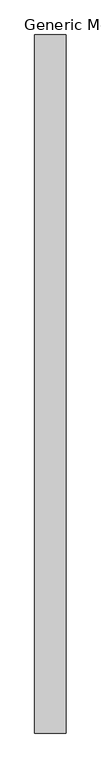
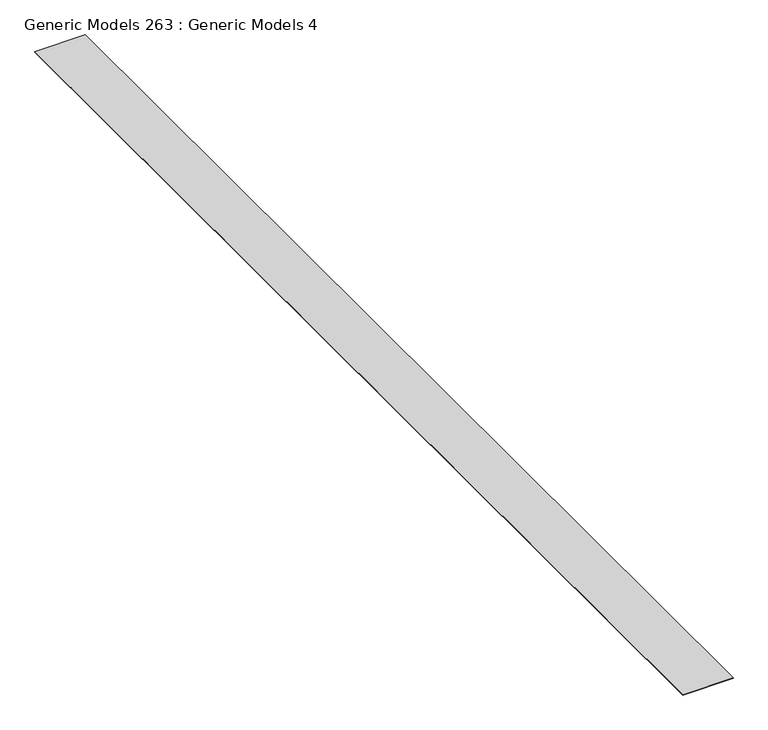
"""IFC4 building model written with IfcOpenShell, lengths in millimetres: proxy geometry, Generic Models 263 : Generic Models 4."""

import ifcopenshell
import ifcopenshell.guid

model = None  # the IFC model being written
_history = None  # IfcOwnerHistory: only IFC2X3 demands one
_inside = {}  # id of a spatial element -> (the spatial element, [elements in it])
_under = {}  # id of a project, library or spatial element -> (it, [spatial elements below it])
_declared = {}  # id of a project -> (the project, [libraries it declares])
_typed = {}  # id of a type object -> (the type object, [elements of that type])
_made_of = {}  # id of a material, layer set ... -> (it, [elements and type objects made of it])


def new_model(schema):
    """Start an empty IFC model of exactly this schema.

    Asked for "IFC4X3", IfcOpenShell would pick the latest addendum, in which some entities
    have other attributes; the version numbers below select the first issue.
    IFC2X3 requires an IfcOwnerHistory on every rooted entity: one is made here for all.
    """
    global model, _history
    if schema == "IFC4X3":
        model = ifcopenshell.file(schema_version=(4, 3, 0, 0))
    else:
        model = ifcopenshell.file(schema=schema)
    _inside.clear()
    _under.clear()
    _declared.clear()
    _typed.clear()
    _made_of.clear()
    _history = None
    if model.schema == "IFC2X3":
        org = make("IfcOrganization", Name="unknown")
        user = make(
            "IfcPersonAndOrganization",
            ThePerson=make("IfcPerson", FamilyName="unknown"),
            TheOrganization=org,
        )
        app = make(
            "IfcApplication",
            ApplicationDeveloper=org,
            Version="unknown",
            ApplicationFullName="unknown",
            ApplicationIdentifier="unknown",
        )
        _history = make(
            "IfcOwnerHistory",
            OwningUser=user,
            OwningApplication=app,
            ChangeAction="ADDED",
            CreationDate=0,
        )
    return model


def make(cls, **values):
    """One entity of the class cls with the attributes given. An attribute that is None is left unset."""
    return model.create_entity(
        cls, **{name: value for name, value in values.items() if value is not None}
    )


def rooted(cls, **values):
    """An entity with a GlobalId (a new one), such as an element, a storey or a relation."""
    return make(cls, GlobalId=ifcopenshell.guid.new(), OwnerHistory=_history, **values)


def si_unit(unit_type, name, prefix=None):
    """IfcSIUnit, for example si_unit("LENGTHUNIT", "METRE", prefix="MILLI")."""
    return make("IfcSIUnit", UnitType=unit_type, Prefix=prefix, Name=name)


def assignment(units):
    """IfcUnitAssignment: the units of a project."""
    return None if units is None else make("IfcUnitAssignment", Units=units)


def point(xyz):
    """IfcCartesianPoint."""
    return None if xyz is None else make("IfcCartesianPoint", Coordinates=xyz)


def direction(xyz):
    """IfcDirection."""
    return None if xyz is None else make("IfcDirection", DirectionRatios=xyz)


def frame(location, z_axis=None, x_axis=None):
    """IfcAxis2Placement3D, a coordinate frame: its origin and axes. An axis left out is left unset."""
    return make(
        "IfcAxis2Placement3D",
        Location=point(location),
        Axis=direction(z_axis),
        RefDirection=direction(x_axis),
    )


def origin():
    """The frame at (0, 0, 0) with its axes left unset."""
    return frame((0.0, 0.0, 0.0))


def place(relative_to, where):
    """IfcLocalPlacement: puts the frame where relative to a parent placement (None: the world)."""
    return make(
        "IfcLocalPlacement", PlacementRelTo=relative_to, RelativePlacement=where
    )


def context(
    kind, dimensions, precision=None, world=None, true_north=None, identifier=None
):
    """IfcGeometricRepresentationContext, for example the 3D "Model" context."""
    return make(
        "IfcGeometricRepresentationContext",
        ContextIdentifier=identifier,
        ContextType=kind,
        CoordinateSpaceDimension=dimensions,
        Precision=precision,
        WorldCoordinateSystem=world,
        TrueNorth=true_north,
    )


def project(units=None, contexts=None):
    """IfcProject with its units and contexts."""
    return rooted(
        "IfcProject",
        Name="project",
        RepresentationContexts=contexts,
        UnitsInContext=assignment(units),
    )


def spatial(cls, under=None, at=None, **own):
    """A site, building, storey or space (cls), placed at a placement, below another one or the project."""
    s = rooted(cls, ObjectPlacement=at, **own)
    if under is not None:
        _under.setdefault(under.id(), (under, []))[1].append(s)
    return s


def polyline(points):
    """IfcPolyline through the points."""
    return make("IfcPolyline", Points=[point(p) for p in points])


def outline(outer, holes=None, kind="AREA"):
    """IfcArbitraryClosedProfileDef: a profile drawn as a closed curve; with holes, ...WithVoids."""
    if holes is None:
        return make("IfcArbitraryClosedProfileDef", ProfileType=kind, OuterCurve=outer)
    return make(
        "IfcArbitraryProfileDefWithVoids",
        ProfileType=kind,
        OuterCurve=outer,
        InnerCurves=holes,
    )


def extrude(swept, where, along, depth):
    """IfcExtrudedAreaSolid: the profile swept, set in the frame where, extruded along a direction by depth."""
    return make(
        "IfcExtrudedAreaSolid",
        SweptArea=swept,
        Position=where,
        ExtrudedDirection=direction(along),
        Depth=depth,
    )


def shape(context_of_items, identifier, shape_type, items):
    """IfcShapeRepresentation: the items that make up one representation, for example the "Body"."""
    return make(
        "IfcShapeRepresentation",
        ContextOfItems=context_of_items,
        RepresentationIdentifier=identifier,
        RepresentationType=shape_type,
        Items=items,
    )


def source(mapping_origin, context_of_items, identifier, shape_type, items):
    """IfcRepresentationMap: a shape defined once, which mapped items show again and again."""
    return make(
        "IfcRepresentationMap",
        MappingOrigin=mapping_origin,
        MappedRepresentation=shape(context_of_items, identifier, shape_type, items),
    )


def transform(
    local_origin,
    x_axis=None,
    y_axis=None,
    z_axis=None,
    scale=None,
    scale2=None,
    scale3=None,
    uniform=True,
):
    """IfcCartesianTransformationOperator3D, or its non-uniform kind. x_axis, y_axis, z_axis: its Axis1, 2, 3."""
    if uniform:
        return make(
            "IfcCartesianTransformationOperator3D",
            Axis1=direction(x_axis),
            Axis2=direction(y_axis),
            LocalOrigin=point(local_origin),
            Scale=scale,
            Axis3=direction(z_axis),
        )
    return make(
        "IfcCartesianTransformationOperator3DnonUniform",
        Axis1=direction(x_axis),
        Axis2=direction(y_axis),
        LocalOrigin=point(local_origin),
        Scale=scale,
        Axis3=direction(z_axis),
        Scale2=scale2,
        Scale3=scale3,
    )


def mapped(mapping_source, mapping_target):
    """IfcMappedItem: shows the shape of a source again, moved by a transform."""
    return make(
        "IfcMappedItem", MappingSource=mapping_source, MappingTarget=mapping_target
    )


def made_of(thing, what):
    """Note that an element or type object is made of a material, layer set ...; save() writes the relation."""
    if what is not None:
        _made_of.setdefault(what.id(), (what, []))[1].append(thing)
    return thing


def element(
    cls,
    number,
    at=None,
    inside=None,
    cuts=None,
    type_object=None,
    material=None,
    context=None,
    identifier="Body",
    shape_type=None,
    held_by="IfcProductDefinitionShape",
    body=None,
    shapes=None,
    **own,
):
    """One element of the class cls, such as IfcWall. Its Tag is "e" and its number.

    at: its placement. inside: the storey or other place that contains it. cuts: it is an
    opening in that element (IfcRelVoidsElement). A single representation is given by context,
    identifier, shape_type and body (its items); several are given by shapes. held_by: the class
    of the entity that holds the representations. save() writes the other relations.
    """
    e = rooted(cls, Tag="e%d" % number, ObjectPlacement=at, **own)
    if body is not None:
        shapes = [shape(context, identifier, shape_type, body)]
    if shapes is not None:
        e.Representation = make(held_by, Representations=shapes)
    if inside is not None:
        _inside.setdefault(inside.id(), (inside, []))[1].append(e)
    if cuts is not None:
        rooted(
            "IfcRelVoidsElement", RelatingBuildingElement=cuts, RelatedOpeningElement=e
        )
    if type_object is not None:
        _typed.setdefault(type_object.id(), (type_object, []))[1].append(e)
    return made_of(e, material)


def aggregate(whole, parts):
    """IfcRelAggregates: a whole, such as a stair, and the parts it consists of."""
    return rooted("IfcRelAggregates", RelatingObject=whole, RelatedObjects=parts)


def save(model, path):
    """Write the relations noted so far, then the file.

    IfcRelAggregates (storeys below a building ...), IfcRelContainedInSpatialStructure (elements
    in a storey), IfcRelDefinesByType, IfcRelAssociatesMaterial and IfcRelDeclares: one each for
    every whole, place, type object, material and project.
    """
    for whole, parts in _under.values():
        aggregate(whole, parts)
    for where, things in _inside.values():
        rooted(
            "IfcRelContainedInSpatialStructure",
            RelatedElements=things,
            RelatingStructure=where,
        )
    for kind, things in _typed.values():
        rooted("IfcRelDefinesByType", RelatedObjects=things, RelatingType=kind)
    for what, things in _made_of.values():
        rooted("IfcRelAssociatesMaterial", RelatedObjects=things, RelatingMaterial=what)
    for by, libraries in _declared.values():
        rooted("IfcRelDeclares", RelatingContext=by, RelatedDefinitions=libraries)
    model.write(path)


def generic_models_263_generic_models_4_84147d02(model_context):
    return source(origin(), model_context, "Body", "SweptSolid", [
        extrude(outline(polyline([(1515.5714201, -5493.3230338), (951.0479772, -5493.3230338), (951.0479772, 7054.2769662), (1515.5714201, 7054.2769662), (1515.5714201, -5493.3230338)])), frame((0.0, 0.0, 123435.8085), z_axis=(0.0, 0.0, 1.0), x_axis=(1.0, 0.0, 0.0)), (0.0, 0.0, 1.0), 4.7625),
    ])


if __name__ == "__main__":
    model = new_model("IFC4")
    model_context = context("Model", 3, world=origin())
    ifc_project = project(units=[si_unit("LENGTHUNIT", "METRE", prefix="MILLI")], contexts=[model_context])
    site = spatial("IfcSite", under=ifc_project)
    building = spatial("IfcBuilding", under=site)
    placement = place(None, origin())
    generic_models_263_generic_models_4_shape = generic_models_263_generic_models_4_84147d02(model_context)
    element("IfcBuildingElementProxy", 1, Name="Generic Models 263 : Generic Models 4", ObjectType="Generic Models 263 : Generic Models 4", at=placement, inside=building, context=model_context, shape_type="MappedRepresentation", body=[
        mapped(generic_models_263_generic_models_4_shape, transform((0.0, 0.0, 0.0), x_axis=(1.0, 0.0, 0.0), y_axis=(0.0, 1.0, 0.0), z_axis=(0.0, 0.0, 1.0))),
    ])
    save(model, "model.ifc")

# Revit data of these elements
# Element 1 (IfcBuildingElementProxy, "Generic Models 263 : Generic Models 4")
#   Materials on its faces: "_MORTAR SETTING BED"
# Materials
#   "_MORTAR SETTING BED": class "Generic", colour RGB 191 191 191, transparency 0, Cost = 0
